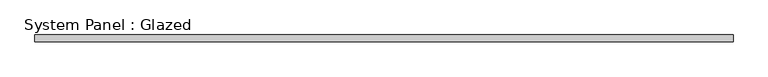
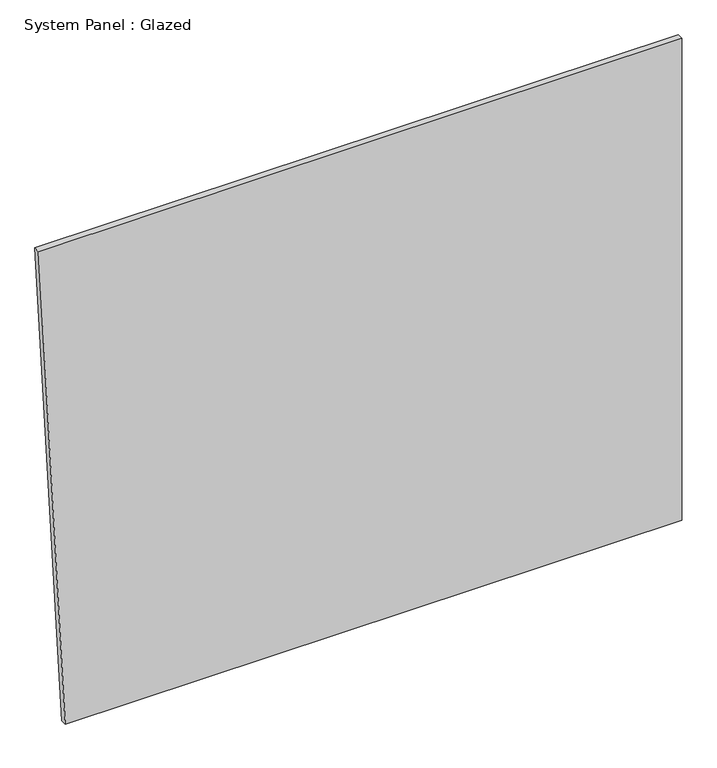
"""IFC4 building model written with IfcOpenShell, lengths in millimetres: plate geometry, System Panel : Glazed."""

import ifcopenshell
import ifcopenshell.guid

model = None  # the IFC model being written
_history = None  # IfcOwnerHistory: only IFC2X3 demands one
_inside = {}  # id of a spatial element -> (the spatial element, [elements in it])
_under = {}  # id of a project, library or spatial element -> (it, [spatial elements below it])
_declared = {}  # id of a project -> (the project, [libraries it declares])
_typed = {}  # id of a type object -> (the type object, [elements of that type])
_made_of = {}  # id of a material, layer set ... -> (it, [elements and type objects made of it])


def new_model(schema):
    """Start an empty IFC model of exactly this schema.

    Asked for "IFC4X3", IfcOpenShell would pick the latest addendum, in which some entities
    have other attributes; the version numbers below select the first issue.
    IFC2X3 requires an IfcOwnerHistory on every rooted entity: one is made here for all.
    """
    global model, _history
    if schema == "IFC4X3":
        model = ifcopenshell.file(schema_version=(4, 3, 0, 0))
    else:
        model = ifcopenshell.file(schema=schema)
    _inside.clear()
    _under.clear()
    _declared.clear()
    _typed.clear()
    _made_of.clear()
    _history = None
    if model.schema == "IFC2X3":
        org = make("IfcOrganization", Name="unknown")
        user = make(
            "IfcPersonAndOrganization",
            ThePerson=make("IfcPerson", FamilyName="unknown"),
            TheOrganization=org,
        )
        app = make(
            "IfcApplication",
            ApplicationDeveloper=org,
            Version="unknown",
            ApplicationFullName="unknown",
            ApplicationIdentifier="unknown",
        )
        _history = make(
            "IfcOwnerHistory",
            OwningUser=user,
            OwningApplication=app,
            ChangeAction="ADDED",
            CreationDate=0,
        )
    return model


def make(cls, **values):
    """One entity of the class cls with the attributes given. An attribute that is None is left unset."""
    return model.create_entity(
        cls, **{name: value for name, value in values.items() if value is not None}
    )


def rooted(cls, **values):
    """An entity with a GlobalId (a new one), such as an element, a storey or a relation."""
    return make(cls, GlobalId=ifcopenshell.guid.new(), OwnerHistory=_history, **values)


def si_unit(unit_type, name, prefix=None):
    """IfcSIUnit, for example si_unit("LENGTHUNIT", "METRE", prefix="MILLI")."""
    return make("IfcSIUnit", UnitType=unit_type, Prefix=prefix, Name=name)


def assignment(units):
    """IfcUnitAssignment: the units of a project."""
    return None if units is None else make("IfcUnitAssignment", Units=units)


def point(xyz):
    """IfcCartesianPoint."""
    return None if xyz is None else make("IfcCartesianPoint", Coordinates=xyz)


def direction(xyz):
    """IfcDirection."""
    return None if xyz is None else make("IfcDirection", DirectionRatios=xyz)


def frame(location, z_axis=None, x_axis=None):
    """IfcAxis2Placement3D, a coordinate frame: its origin and axes. An axis left out is left unset."""
    return make(
        "IfcAxis2Placement3D",
        Location=point(location),
        Axis=direction(z_axis),
        RefDirection=direction(x_axis),
    )


def origin():
    """The frame at (0, 0, 0) with its axes left unset."""
    return frame((0.0, 0.0, 0.0))


def place(relative_to, where):
    """IfcLocalPlacement: puts the frame where relative to a parent placement (None: the world)."""
    return make(
        "IfcLocalPlacement", PlacementRelTo=relative_to, RelativePlacement=where
    )


def context(
    kind, dimensions, precision=None, world=None, true_north=None, identifier=None
):
    """IfcGeometricRepresentationContext, for example the 3D "Model" context."""
    return make(
        "IfcGeometricRepresentationContext",
        ContextIdentifier=identifier,
        ContextType=kind,
        CoordinateSpaceDimension=dimensions,
        Precision=precision,
        WorldCoordinateSystem=world,
        TrueNorth=true_north,
    )


def project(units=None, contexts=None):
    """IfcProject with its units and contexts."""
    return rooted(
        "IfcProject",
        Name="project",
        RepresentationContexts=contexts,
        UnitsInContext=assignment(units),
    )


def spatial(cls, under=None, at=None, **own):
    """A site, building, storey or space (cls), placed at a placement, below another one or the project."""
    s = rooted(cls, ObjectPlacement=at, **own)
    if under is not None:
        _under.setdefault(under.id(), (under, []))[1].append(s)
    return s


def polyline(points):
    """IfcPolyline through the points."""
    return make("IfcPolyline", Points=[point(p) for p in points])


def outline(outer, holes=None, kind="AREA"):
    """IfcArbitraryClosedProfileDef: a profile drawn as a closed curve; with holes, ...WithVoids."""
    if holes is None:
        return make("IfcArbitraryClosedProfileDef", ProfileType=kind, OuterCurve=outer)
    return make(
        "IfcArbitraryProfileDefWithVoids",
        ProfileType=kind,
        OuterCurve=outer,
        InnerCurves=holes,
    )


def extrude(swept, where, along, depth):
    """IfcExtrudedAreaSolid: the profile swept, set in the frame where, extruded along a direction by depth."""
    return make(
        "IfcExtrudedAreaSolid",
        SweptArea=swept,
        Position=where,
        ExtrudedDirection=direction(along),
        Depth=depth,
    )


def shape(context_of_items, identifier, shape_type, items):
    """IfcShapeRepresentation: the items that make up one representation, for example the "Body"."""
    return make(
        "IfcShapeRepresentation",
        ContextOfItems=context_of_items,
        RepresentationIdentifier=identifier,
        RepresentationType=shape_type,
        Items=items,
    )


def source(mapping_origin, context_of_items, identifier, shape_type, items):
    """IfcRepresentationMap: a shape defined once, which mapped items show again and again."""
    return make(
        "IfcRepresentationMap",
        MappingOrigin=mapping_origin,
        MappedRepresentation=shape(context_of_items, identifier, shape_type, items),
    )


def transform(
    local_origin,
    x_axis=None,
    y_axis=None,
    z_axis=None,
    scale=None,
    scale2=None,
    scale3=None,
    uniform=True,
):
    """IfcCartesianTransformationOperator3D, or its non-uniform kind. x_axis, y_axis, z_axis: its Axis1, 2, 3."""
    if uniform:
        return make(
            "IfcCartesianTransformationOperator3D",
            Axis1=direction(x_axis),
            Axis2=direction(y_axis),
            LocalOrigin=point(local_origin),
            Scale=scale,
            Axis3=direction(z_axis),
        )
    return make(
        "IfcCartesianTransformationOperator3DnonUniform",
        Axis1=direction(x_axis),
        Axis2=direction(y_axis),
        LocalOrigin=point(local_origin),
        Scale=scale,
        Axis3=direction(z_axis),
        Scale2=scale2,
        Scale3=scale3,
    )


def mapped(mapping_source, mapping_target):
    """IfcMappedItem: shows the shape of a source again, moved by a transform."""
    return make(
        "IfcMappedItem", MappingSource=mapping_source, MappingTarget=mapping_target
    )


def made_of(thing, what):
    """Note that an element or type object is made of a material, layer set ...; save() writes the relation."""
    if what is not None:
        _made_of.setdefault(what.id(), (what, []))[1].append(thing)
    return thing


def element(
    cls,
    number,
    at=None,
    inside=None,
    cuts=None,
    type_object=None,
    material=None,
    context=None,
    identifier="Body",
    shape_type=None,
    held_by="IfcProductDefinitionShape",
    body=None,
    shapes=None,
    **own,
):
    """One element of the class cls, such as IfcWall. Its Tag is "e" and its number.

    at: its placement. inside: the storey or other place that contains it. cuts: it is an
    opening in that element (IfcRelVoidsElement). A single representation is given by context,
    identifier, shape_type and body (its items); several are given by shapes. held_by: the class
    of the entity that holds the representations. save() writes the other relations.
    """
    e = rooted(cls, Tag="e%d" % number, ObjectPlacement=at, **own)
    if body is not None:
        shapes = [shape(context, identifier, shape_type, body)]
    if shapes is not None:
        e.Representation = make(held_by, Representations=shapes)
    if inside is not None:
        _inside.setdefault(inside.id(), (inside, []))[1].append(e)
    if cuts is not None:
        rooted(
            "IfcRelVoidsElement", RelatingBuildingElement=cuts, RelatedOpeningElement=e
        )
    if type_object is not None:
        _typed.setdefault(type_object.id(), (type_object, []))[1].append(e)
    return made_of(e, material)


def aggregate(whole, parts):
    """IfcRelAggregates: a whole, such as a stair, and the parts it consists of."""
    return rooted("IfcRelAggregates", RelatingObject=whole, RelatedObjects=parts)


def save(model, path):
    """Write the relations noted so far, then the file.

    IfcRelAggregates (storeys below a building ...), IfcRelContainedInSpatialStructure (elements
    in a storey), IfcRelDefinesByType, IfcRelAssociatesMaterial and IfcRelDeclares: one each for
    every whole, place, type object, material and project.
    """
    for whole, parts in _under.values():
        aggregate(whole, parts)
    for where, things in _inside.values():
        rooted(
            "IfcRelContainedInSpatialStructure",
            RelatedElements=things,
            RelatingStructure=where,
        )
    for kind, things in _typed.values():
        rooted("IfcRelDefinesByType", RelatedObjects=things, RelatingType=kind)
    for what, things in _made_of.values():
        rooted("IfcRelAssociatesMaterial", RelatedObjects=things, RelatingMaterial=what)
    for by, libraries in _declared.values():
        rooted("IfcRelDeclares", RelatingContext=by, RelatedDefinitions=libraries)
    model.write(path)


def system_panel_glazed_e0da27cb(model_context):
    return source(origin(), model_context, "Body", "SweptSolid", [
        extrude(outline(polyline([(0.0, -1208.7338763), (0.0, 1317.8741594), (2085.3785982, 1317.8741594), (2085.3785982, -1317.8741594), (0.0, -1208.7338763)])), frame((0.0, -44.45, 0.0), z_axis=(0.0, 1.0, 0.0), x_axis=(0.0, 0.0, 1.0)), (0.0, 0.0, 1.0), 25.4),
    ])


if __name__ == "__main__":
    model = new_model("IFC4")
    model_context = context("Model", 3, world=origin())
    ifc_project = project(units=[si_unit("LENGTHUNIT", "METRE", prefix="MILLI")], contexts=[model_context])
    site = spatial("IfcSite", under=ifc_project)
    building = spatial("IfcBuilding", under=site)
    placement = place(None, origin())
    system_panel_glazed_shape = system_panel_glazed_e0da27cb(model_context)
    element("IfcPlate", 1, ObjectType="System Panel : Glazed", at=placement, inside=building, context=model_context, shape_type="MappedRepresentation", body=[
        mapped(system_panel_glazed_shape, transform((0.0, 0.0, 0.0), x_axis=(1.0, 0.0, 0.0), y_axis=(0.0, 1.0, 0.0), z_axis=(0.0, 0.0, 1.0))),
    ])
    save(model, "model.ifc")

# Revit data of these elements
# Type "System Panel : Glazed"
#   Construction Type Id = "GSP4R"
#   Analytic Construction = "1/8 in Pilkington single glazing"
#   Visual Light Transmittance = 0.9
#   Solar Heat Gain Coefficient = 0.86
#   Heat Transfer Coefficient (U) = 1.18115 BTU/(h·ft²·°F)
#   Define Thermal Properties by = 1
# Element 1 (IfcPlate, "System Panel : Glazed")
#   Materials on its faces: "Glass"
# Materials
#   "Glass": class "Glass", colour RGB 0 128 192, transparency 0.75, Description = "Soda Lime Glass", Cost = 0
